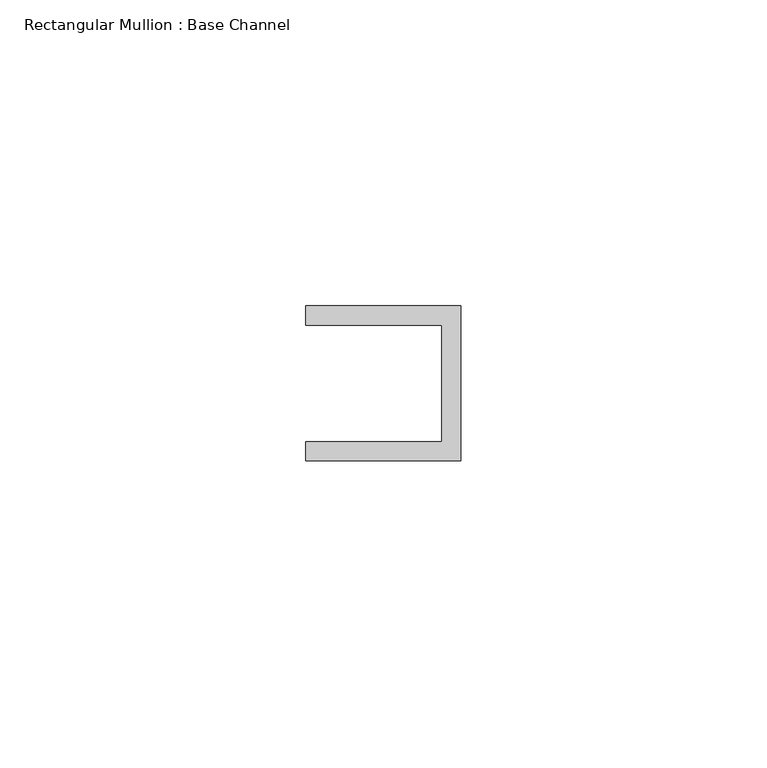
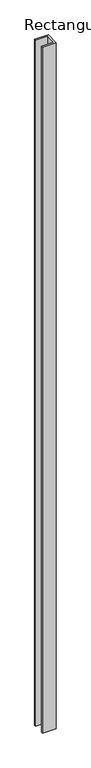
"""IFC4 building model written with IfcOpenShell, lengths in millimetres: member geometry, Rectangular Mullion : Base Channel."""

from ifc_helpers import new_model, si_unit, frame, origin, place, context, project, spatial, polyline, outline, extrude, source, transform, mapped, element, save


def rectangular_mullion_base_channel_b39aeb49(model_context):
    return source(origin(), model_context, "Body", "SweptSolid", [
        extrude(outline(polyline([(0.0, 12.7), (0.0, -12.7), (-25.4, -12.7), (-25.4, -9.525), (-3.175, -9.525), (-3.175, 9.525), (-25.4, 9.525), (-25.4, 12.7), (0.0, 12.7)])), frame((0.0, 0.0, -1352.55), z_axis=(0.0, 0.0, 1.0), x_axis=(1.0, 0.0, 0.0)), (0.0, 0.0, 1.0), 1352.55),
    ])


if __name__ == "__main__":
    model = new_model("IFC4")
    model_context = context("Model", 3, world=origin())
    ifc_project = project(units=[si_unit("LENGTHUNIT", "METRE", prefix="MILLI")], contexts=[model_context])
    site = spatial("IfcSite", under=ifc_project)
    building = spatial("IfcBuilding", under=site)
    placement = place(None, origin())
    rectangular_mullion_base_channel_shape = rectangular_mullion_base_channel_b39aeb49(model_context)
    element("IfcMember", 1, ObjectType="Rectangular Mullion : Base Channel", at=placement, inside=building, context=model_context, shape_type="MappedRepresentation", body=[
        mapped(rectangular_mullion_base_channel_shape, transform((0.0, 0.0, 0.0), x_axis=(1.0, 0.0, 0.0), y_axis=(0.0, 1.0, 0.0), z_axis=(0.0, 0.0, 1.0))),
    ])
    save(model, "model.ifc")

# Revit data of these elements
# Type "Rectangular Mullion : Base Channel"
#   built-in parameter 1007322 = 0.0833333 (stored number, unit not read)
#   built-in parameter 1007321 = 0.0416667 (stored number, unit not read)
#   built-in parameter 1007320 = -0.03125 (stored number, unit not read)
# Element 1 (IfcMember, "Rectangular Mullion : Base Channel")
#   Materials on its faces: "ALUM"
# Materials
#   "ALUM": class "Generic", colour RGB 157 157 157, transparency 0, Cost = 0
